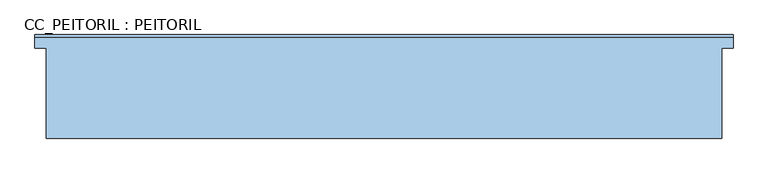
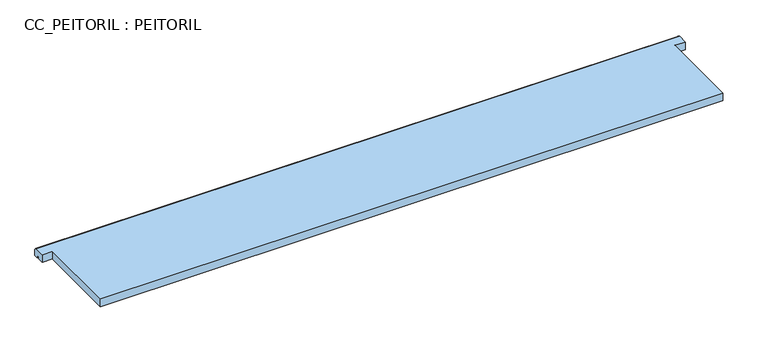
"""IFC4 building model written with IfcOpenShell, lengths in millimetres: window geometry, CC_PEITORIL : PEITORIL."""

from ifc_helpers import new_model, si_unit, frame, origin, place, context, project, spatial, circle_curve, source, transform, mapped, element, save
from ifc_brep_helpers import plane_surface, cylinder_surface, advanced_brep


def cc_peitoril_peitoril_5741519e(model_context):
    return source(origin(), model_context, "Body", "AdvancedBrep", [
        advanced_brep(
        [(-750.0, 100.0, 1500.0), (-750.0, -100.0, 1500.0), (750.0, -100.0, 1500.0), (750.0, 100.0, 1500.0), (775.0, 100.0, 1500.0), (775.0, 123.4916648, 1500.0), (-775.0, 123.4916648, 1500.0), (-775.0, 100.0, 1500.0), (-750.0, 100.0, 1480.0), (-775.0, 100.0, 1480.0), (-775.0, 115.0, 1480.0), (775.0, 115.0, 1480.0), (775.0, 100.0, 1480.0), (750.0, 100.0, 1480.0), (750.0, -100.0, 1480.0), (-750.0, -100.0, 1480.0), (-775.0, 130.0, 1480.0), (775.0, 130.0, 1480.0), (775.0, 120.0, 1480.0), (-775.0, 120.0, 1480.0), (775.0, 115.0, 1485.0), (775.0, 120.0, 1485.0), (775.0, 130.0, 1493.4916648), (-775.0, 130.0, 1493.4916648), (-775.0, 120.0, 1485.0), (-775.0, 115.0, 1485.0)],
        [
            (0, 1),
            (1, 2),
            (2, 3),
            (3, 4),
            (4, 5),
            (5, 6),
            (6, 7),
            (7, 0),
            (8, 9),
            (9, 10),
            (10, 11),
            (11, 12),
            (12, 13),
            (13, 14),
            (14, 15),
            (15, 8),
            (16, 17),
            (17, 18),
            (18, 19),
            (19, 16),
            (0, 8),
            (15, 1),
            (14, 2),
            (13, 3),
            (12, 4),
            (11, 20),
            (20, 21),
            (21, 18),
            (17, 22),
            (22, 5, circle_curve(frame((775.0, 123.4916648, 1493.4916648), z_axis=(1.0, 0.0, 0.0), x_axis=(0.0, -1.0, 0.0)), 6.5083352)),
            (16, 23),
            (23, 22),
            (9, 7),
            (6, 23, circle_curve(frame((-775.0, 123.4916648, 1493.4916648), z_axis=(-1.0, 0.0, 0.0), x_axis=(0.0, -1.0, 0.0)), 6.5083352)),
            (19, 24),
            (24, 25),
            (25, 10),
            (24, 21),
            (20, 25),
        ],
        [
            plane_surface(frame((-750.0, -100.0, 1500.0), z_axis=(0.0, 0.0, 1.0), x_axis=(0.0, -1.0, 0.0))),
            plane_surface(frame((-750.0, -100.0, 1480.0), z_axis=(0.0, 0.0, -1.0), x_axis=(0.0, 1.0, 0.0))),
            plane_surface(frame((-750.0, 100.0, 1500.0), z_axis=(-1.0, 0.0, 0.0), x_axis=(0.0, 0.0, -1.0))),
            plane_surface(frame((-750.0, -100.0, 1500.0), z_axis=(0.0, -1.0, 0.0), x_axis=(0.0, 0.0, -1.0))),
            plane_surface(frame((750.0, -100.0, 1500.0), z_axis=(1.0, 0.0, 0.0), x_axis=(0.0, 0.0, -1.0))),
            plane_surface(frame((750.0, 100.0, 1500.0), z_axis=(0.0, -1.0, 0.0), x_axis=(0.0, 0.0, -1.0))),
            plane_surface(frame((775.0, 100.0, 1500.0), z_axis=(1.0, 0.0, 0.0), x_axis=(0.0, 0.0, -1.0))),
            plane_surface(frame((775.0, 130.0, 1500.0), z_axis=(0.0, 1.0, 0.0), x_axis=(0.0, 0.0, -1.0))),
            plane_surface(frame((-775.0, 130.0, 1500.0), z_axis=(-1.0, 0.0, 0.0), x_axis=(0.0, 0.0, -1.0))),
            plane_surface(frame((-775.0, 100.0, 1500.0), z_axis=(0.0, -1.0, 0.0), x_axis=(0.0, 0.0, -1.0))),
            cylinder_surface(frame((775.0, 123.4916648, 1493.4916648), z_axis=(-1.0, 0.0, 0.0), x_axis=(0.0, -1.0, 0.0)), 6.5083352),
            plane_surface(frame((-775.0, 115.0, 1485.0), z_axis=(0.0, 0.0, -1.0), x_axis=(1.0, 0.0, 0.0))),
            plane_surface(frame((-775.0, 120.0, 1485.0), z_axis=(0.0, -1.0, 0.0), x_axis=(1.0, 0.0, 0.0))),
            plane_surface(frame((-775.0, 115.0, 1480.0), z_axis=(0.0, 1.0, 0.0), x_axis=(1.0, 0.0, 0.0))),
        ],
        [
            (0, [[1, 2, 3, 4, 5, 6, 7, 8]]),
            (1, [[9, 10, 11, 12, 13, 14, 15, 16]]),
            (1, [[17, 18, 19, 20]]),
            (2, [[-1, 21, -16, 22]]),
            (3, [[-2, -22, -15, 23]]),
            (4, [[-3, -23, -14, 24]]),
            (5, [[-4, -24, -13, 25]]),
            (6, [[-25, -12, 26, 27, 28, -18, 29, 30, -5]]),
            (7, [[-17, 31, 32, -29]]),
            (8, [[33, -7, 34, -31, -20, 35, 36, 37, -10]]),
            (9, [[-8, -33, -9, -21]]),
            (10, [[-6, -30, -32, -34]]),
            (11, [[38, -27, 39, -36]]),
            (12, [[-38, -35, -19, -28]]),
            (13, [[-39, -26, -11, -37]]),
        ],
    ),
    ])


if __name__ == "__main__":
    model = new_model("IFC4")
    model_context = context("Model", 3, world=origin())
    ifc_project = project(units=[si_unit("LENGTHUNIT", "METRE", prefix="MILLI")], contexts=[model_context])
    site = spatial("IfcSite", under=ifc_project)
    building = spatial("IfcBuilding", under=site)
    placement = place(None, origin())
    cc_peitoril_peitoril_shape = cc_peitoril_peitoril_5741519e(model_context)
    element("IfcWindow", 1, ObjectType="CC_PEITORIL : PEITORIL", at=placement, inside=building, context=model_context, shape_type="MappedRepresentation", body=[
        mapped(cc_peitoril_peitoril_shape, transform((0.0, 0.0, 0.0), x_axis=(1.0, 0.0, 0.0), y_axis=(0.0, 1.0, 0.0), z_axis=(0.0, 0.0, 1.0))),
    ])
    save(model, "model.ifc")

# Revit data of these elements
# Type "CC_PEITORIL : PEITORIL"
#   Type Mark = "PEITORIL"
#   Analytic Construction = "<Nenhum>"
#   Largura da pedra [instance default] = 0.26 m
#   Interna [instance default] = 0.08 m
#   Externa [instance default] = 0.008142 m
#   Extensão Exterior [instance default] = 0.03 m
#   Extensão Exterior Esquerda [instance default] = 0.085058 m
#   Extensão Exterior Direita [instance default] = 0.10 m
#   Espessura [instance default] = 0.02 m
#   Comprimento [instance default] = 1.00 m
#   Altura-padrão do peitoril = 1.48 m
#   ----EXTENSÃO---- [instance default] = 0.00 m
#   ----DEMAIS---- [instance default] = 0.00 m
#   Peitoril [instance default] = none
#   Rough Width = 0
#   Rough Height = 0
#   Height = 0
#   Wall Closure = (empty or 0)
#   Width = 0
# Element 1 (IfcWindow, "CC_PEITORIL : PEITORIL")
#   Interna = 0.00 m
#   Externa = 0.00 m
#   Extensão Exterior Esquerda = 0.025 m
#   Extensão Exterior Direita = 0.025 m
#   Comprimento = 1.50 m
#   Peitoril = .GRANITO BRANCO ITAÚNAS
#   Materials on its faces: ".GRANITO BRANCO ITAÚNAS"
# Materials
#   ".GRANITO BRANCO ITAÚNAS": class ".CC_PEDRA REVEST.", colour RGB 202 195 174, transparency 0, Description = "Granito branco Itaúnas", Uso = "Pedra", Cost = 0
